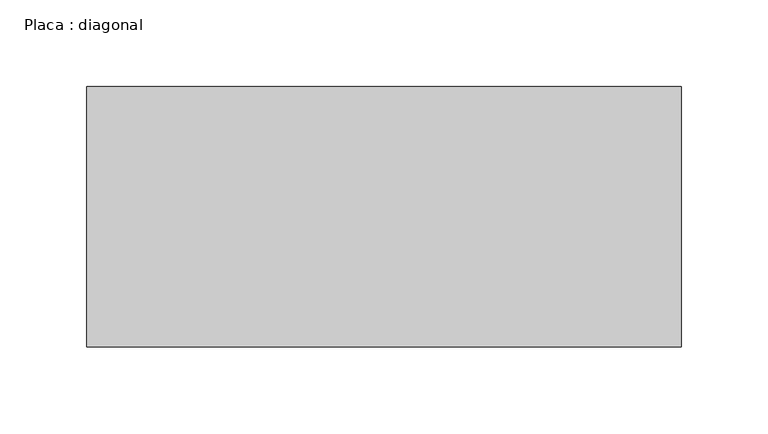
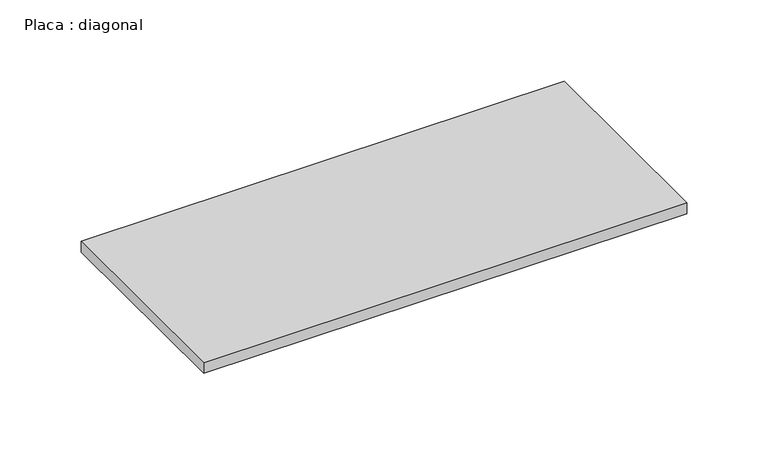
"""IFC4 building model written with IfcOpenShell, lengths in millimetres: beam geometry, Placa : diagonal."""

from ifc_helpers import new_model, si_unit, frame, origin, place, context, project, spatial, polyline, outline, extrude, source, transform, mapped, element, save


def placa_diagonal_982eed0a(model_context):
    return source(origin(), model_context, "Body", "SweptSolid", [
        extrude(outline(polyline([(170.6977727, 75.0), (170.6977727, -75.0), (-171.6122357, -75.0), (-171.6122357, 75.0), (170.6977727, 75.0)])), frame((0.0, 0.0, -4.0), z_axis=(0.0, 0.0, 1.0), x_axis=(1.0, 0.0, 0.0)), (0.0, 0.0, 1.0), 8.0),
    ])


if __name__ == "__main__":
    model = new_model("IFC4")
    model_context = context("Model", 3, world=origin())
    ifc_project = project(units=[si_unit("LENGTHUNIT", "METRE", prefix="MILLI")], contexts=[model_context])
    site = spatial("IfcSite", under=ifc_project)
    building = spatial("IfcBuilding", under=site)
    placement = place(None, origin())
    placa_diagonal_shape = placa_diagonal_982eed0a(model_context)
    element("IfcBeam", 1, ObjectType="Placa : diagonal", at=placement, inside=building, context=model_context, shape_type="MappedRepresentation", body=[
        mapped(placa_diagonal_shape, transform((0.0, 0.0, 0.0), x_axis=(1.0, 0.0, 0.0), y_axis=(0.0, 1.0, 0.0), z_axis=(0.0, 0.0, 1.0))),
    ])
    save(model, "model.ifc")

# Revit data of these elements
# Type "Placa : diagonal"
#   W = 0
#   Length [instance default] = 1.50 m
#   b = 0.15 m
#   d = 0.008 m
#   A = 0 m²
#   Structural Material [instance default] = Aço, 45-345
# Element 1 (IfcBeam, "Placa : diagonal")
#   Materials on its faces: "Aço, 45-345"
# Materials
#   "Aço, 45-345": class "Metal", colour RGB 247 247 247, transparency 0, Description = "Aço 345 MPa", Cost = 0
